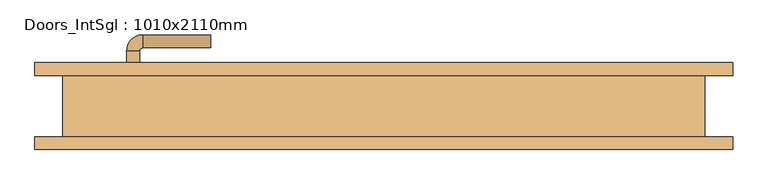
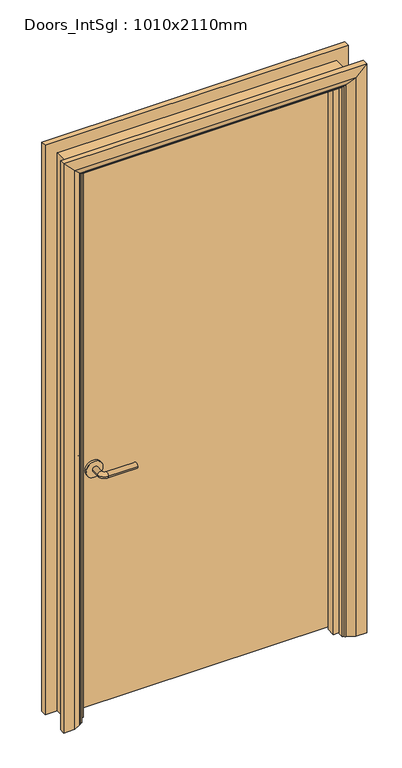
"""IFC4 building model written with IfcOpenShell, lengths in millimetres: door geometry, Doors_IntSgl : 1010x2110mm."""

from ifc_helpers import new_model, si_unit, point, frame, frame_2d, origin, place, context, project, spatial, polyline, circle_curve, ellipse_curve, trimmed, segment, composite_curve, outline, extrude, faceted_brep, source, transform, mapped, element, save
from ifc_brep_helpers import plane_surface, cylinder_surface, revolved_surface, advanced_brep


def doors_intsgl_1010x2110mm_9b3ab836(model_context):
    return source(origin(), model_context, "Body", "SolidModel", [
        advanced_brep(
        [(-398.0, 1.5, 900.0), (-378.0, 1.5, 900.0), (-378.0, -28.5, 900.0), (-398.0, -28.5, 900.0), (-373.0, -33.5, 900.0), (-373.0, -53.5, 900.0), (-268.0, -53.5, 900.0), (-268.0, -33.5, 900.0)],
        [
            (0, 1, circle_curve(frame((-388.0, 1.5, 900.0), z_axis=(0.0, 1.0, 0.0), x_axis=(1.0, 0.0, 0.0)), 10.0)),
            (1, 0, circle_curve(frame((-388.0, 1.5, 900.0), z_axis=(0.0, 1.0, 0.0), x_axis=(1.0, 0.0, 0.0)), 10.0)),
            (1, 2),
            (2, 3, circle_curve(frame((-388.0, -28.5, 900.0), z_axis=(0.0, 1.0, 0.0), x_axis=(1.0, 0.0, 0.0)), 10.0)),
            (3, 0),
            (3, 2, circle_curve(frame((-388.0, -28.5, 900.0), z_axis=(0.0, 1.0, 0.0), x_axis=(1.0, 0.0, 0.0)), 10.0)),
            (4, 5, circle_curve(frame((-373.0, -43.5, 900.0), z_axis=(-1.0, 0.0, 0.0), x_axis=(0.0, 1.0, 0.0)), 10.0)),
            (5, 3, circle_curve(frame((-373.0, -28.5, 900.0), z_axis=(0.0, 0.0, -1.0), x_axis=(-1.0, 0.0, 0.0)), 25.0)),
            (2, 4, circle_curve(frame((-373.0, -28.5, 900.0), z_axis=(0.0, 0.0, 1.0), x_axis=(-1.0, 0.0, 0.0)), 5.0)),
            (5, 4, circle_curve(frame((-373.0, -43.5, 900.0), z_axis=(-1.0, 0.0, 0.0), x_axis=(0.0, 1.0, 0.0)), 10.0)),
            (6, 7, circle_curve(frame((-268.0, -43.5, 900.0), z_axis=(1.0, 0.0, 0.0), x_axis=(0.0, 1.0, 0.0)), 10.0)),
            (7, 6, circle_curve(frame((-268.0, -43.5, 900.0), z_axis=(1.0, 0.0, 0.0), x_axis=(0.0, 1.0, 0.0)), 10.0)),
            (4, 7),
            (6, 5),
        ],
        [
            plane_surface(frame((-388.0, 1.5, 900.0), z_axis=(0.0, 1.0, 0.0), x_axis=(0.0, 0.0, 1.0))),
            cylinder_surface(frame((-388.0, 1.5, 900.0), z_axis=(0.0, 1.0, 0.0), x_axis=(1.0, 0.0, 0.0)), 10.0),
            revolved_surface(trimmed(ellipse_curve(frame((-388.0, -28.5, 900.0), z_axis=(0.0, -1.0, 0.0), x_axis=(1.0, 0.0, 0.0)), 10.0, 10.0), [point((-398.0, -28.5, 900.0))], [point((-378.0, -28.5, 900.0))], True, "CARTESIAN"), (-373.0, -28.5, 900.0), (0.0, 0.0, -1.0)),
            revolved_surface(trimmed(ellipse_curve(frame((-388.0, -28.5, 900.0), z_axis=(0.0, -1.0, 0.0), x_axis=(1.0, 0.0, 0.0)), 10.0, 10.0), [point((-378.0, -28.5, 900.0))], [point((-398.0, -28.5, 900.0))], True, "CARTESIAN"), (-373.0, -28.5, 900.0), (0.0, 0.0, -1.0)),
            plane_surface(frame((-268.0, -43.5, 900.0), z_axis=(1.0, 0.0, 0.0), x_axis=(0.0, 0.0, 1.0))),
            cylinder_surface(frame((-373.0, -43.5, 900.0), z_axis=(-1.0, 0.0, 0.0), x_axis=(0.0, 1.0, 0.0)), 10.0),
        ],
        [
            (0, [[1, 2]]),
            (1, [[3, 4, 5, -2]]),
            (1, [[-5, 6, -3, -1]]),
            (2, [[7, 8, -4, 9]]),
            (3, [[10, -9, -6, -8]]),
            (4, [[11, 12]]),
            (5, [[13, -11, 14, -7]]),
            (5, [[-14, -12, -13, -10]]),
        ],
    ),
        extrude(outline(composite_curve([segment(trimmed(circle_curve(frame_2d((900.0, -390.5)), 30.0), [point((900.0, -420.5))], [point((900.0, -360.5))], False, "CARTESIAN"), True, "CONTINUOUS"), segment(trimmed(circle_curve(frame_2d((900.0, -390.5)), 30.0), [point((900.0, -360.5))], [point((900.0, -420.5))], False, "CARTESIAN"), True, "CONTINUOUS")], self_intersect=False)), frame((0.0, 1.5, 0.0), z_axis=(0.0, 1.0, 0.0), x_axis=(0.0, 0.0, 1.0)), (0.0, 0.0, 1.0), 8.0),
        advanced_brep(
        [(-398.0, 55.5, 900.0), (-378.0, 55.5, 900.0), (-398.0, 85.5, 900.0), (-378.0, 85.5, 900.0), (-373.0, 90.5, 900.0), (-373.0, 110.5, 900.0), (-268.0, 110.5, 900.0), (-268.0, 90.5, 900.0)],
        [
            (0, 1, circle_curve(frame((-388.0, 55.5, 900.0), z_axis=(0.0, -1.0, 0.0), x_axis=(1.0, 0.0, 0.0)), 10.0)),
            (1, 0, circle_curve(frame((-388.0, 55.5, 900.0), z_axis=(0.0, -1.0, 0.0), x_axis=(1.0, 0.0, 0.0)), 10.0)),
            (0, 2),
            (2, 3, circle_curve(frame((-388.0, 85.5, 900.0), z_axis=(0.0, -1.0, 0.0), x_axis=(1.0, 0.0, 0.0)), 10.0)),
            (3, 1),
            (3, 2, circle_curve(frame((-388.0, 85.5, 900.0), z_axis=(0.0, -1.0, 0.0), x_axis=(1.0, 0.0, 0.0)), 10.0)),
            (4, 3, circle_curve(frame((-373.0, 85.5, 900.0), z_axis=(0.0, 0.0, 1.0), x_axis=(-1.0, 0.0, 0.0)), 5.0)),
            (2, 5, circle_curve(frame((-373.0, 85.5, 900.0), z_axis=(0.0, 0.0, -1.0), x_axis=(-1.0, 0.0, 0.0)), 25.0)),
            (5, 4, circle_curve(frame((-373.0, 100.5, 900.0), z_axis=(-1.0, 0.0, 0.0), x_axis=(0.0, -1.0, 0.0)), 10.0)),
            (4, 5, circle_curve(frame((-373.0, 100.5, 900.0), z_axis=(-1.0, 0.0, 0.0), x_axis=(0.0, -1.0, 0.0)), 10.0)),
            (6, 7, circle_curve(frame((-268.0, 100.5, 900.0), z_axis=(1.0, 0.0, 0.0), x_axis=(0.0, -1.0, 0.0)), 10.0)),
            (7, 6, circle_curve(frame((-268.0, 100.5, 900.0), z_axis=(1.0, 0.0, 0.0), x_axis=(0.0, -1.0, 0.0)), 10.0)),
            (5, 6),
            (7, 4),
        ],
        [
            plane_surface(frame((-388.0, 55.5, 900.0), z_axis=(0.0, -1.0, 0.0), x_axis=(0.0, 0.0, 1.0))),
            cylinder_surface(frame((-388.0, 55.5, 900.0), z_axis=(0.0, -1.0, 0.0), x_axis=(1.0, 0.0, 0.0)), 10.0),
            revolved_surface(trimmed(ellipse_curve(frame((-388.0, 85.5, 900.0), z_axis=(0.0, -1.0, 0.0), x_axis=(1.0, 0.0, 0.0)), 10.0, 10.0), [point((-398.0, 85.5, 900.0))], [point((-378.0, 85.5, 900.0))], True, "CARTESIAN"), (-373.0, 85.5, 900.0), (0.0, 0.0, -1.0)),
            revolved_surface(trimmed(ellipse_curve(frame((-388.0, 85.5, 900.0), z_axis=(0.0, -1.0, 0.0), x_axis=(1.0, 0.0, 0.0)), 10.0, 10.0), [point((-378.0, 85.5, 900.0))], [point((-398.0, 85.5, 900.0))], True, "CARTESIAN"), (-373.0, 85.5, 900.0), (0.0, 0.0, -1.0)),
            plane_surface(frame((-268.0, 100.5, 900.0), z_axis=(1.0, 0.0, 0.0), x_axis=(0.0, 0.0, 1.0))),
            cylinder_surface(frame((-373.0, 100.5, 900.0), z_axis=(-1.0, 0.0, 0.0), x_axis=(0.0, -1.0, 0.0)), 10.0),
        ],
        [
            (0, [[1, 2]]),
            (1, [[-1, 3, 4, 5]]),
            (1, [[-2, -5, 6, -3]]),
            (2, [[7, -4, 8, 9]]),
            (3, [[-8, -6, -7, 10]]),
            (4, [[11, 12]]),
            (5, [[-9, 13, -12, 14]]),
            (5, [[-10, -14, -11, -13]]),
        ],
    ),
        extrude(outline(composite_curve([segment(trimmed(circle_curve(frame_2d((900.0, -390.5)), 30.0), [point((900.0, -420.5))], [point((900.0, -360.5))], False, "CARTESIAN"), True, "CONTINUOUS"), segment(trimmed(circle_curve(frame_2d((900.0, -390.5)), 30.0), [point((900.0, -360.5))], [point((900.0, -420.5))], False, "CARTESIAN"), True, "CONTINUOUS")], self_intersect=False)), frame((0.0, 47.5, 0.0), z_axis=(0.0, 1.0, 0.0), x_axis=(0.0, 0.0, 1.0)), (0.0, 0.0, 1.0), 8.0),
        extrude(outline(polyline([(463.0, 9.5), (-463.0, 9.5), (-463.0, 47.5), (463.0, 47.5), (463.0, 9.5)])), frame((0.0, 0.0, 8.0), z_axis=(0.0, 0.0, 1.0), x_axis=(1.0, 0.0, 0.0)), (0.0, 0.0, 1.0), 2060.0),
        advanced_brep(
        [(540.0, 67.5, 0.0), (540.0, 47.5, 0.0), (470.0, 47.5, 0.0), (474.0, 53.5, 0.0), (500.0, 67.5, 0.0), (540.0, 67.5, 2145.0), (540.0, 47.5, 2145.0), (-540.0, 47.5, 2145.0), (-540.0, 47.5, 0.0), (-470.0, 47.5, 0.0), (-470.0, 47.5, 2075.0), (470.0, 47.5, 2075.0), (474.0, 53.5, 2079.0), (500.0, 67.5, 2105.0), (-500.0, 67.5, 2105.0), (-500.0, 67.5, 0.0), (-540.0, 67.5, 0.0), (-540.0, 67.5, 2145.0), (-474.0, 53.5, 2079.0), (-474.0, 53.5, 0.0)],
        [
            (0, 1),
            (1, 2),
            (2, 3, circle_curve(frame((478.0, 46.5, 0.0), z_axis=(0.0, 0.0, -1.0), x_axis=(1.0, 0.0, 0.0)), 8.0622577)),
            (3, 4),
            (4, 0),
            (0, 5),
            (5, 6),
            (6, 1),
            (6, 7),
            (7, 8),
            (8, 9),
            (9, 10),
            (10, 11),
            (11, 2),
            (11, 12, ellipse_curve(frame((478.0, 46.5, 2083.0), z_axis=(0.7071067811865475, 0.0, -0.7071067811865475), x_axis=(-0.7071067811865474, 0.0, -0.7071067811865476)), 11.4017543, 8.0622577)),
            (12, 3),
            (12, 13),
            (13, 4),
            (13, 14),
            (14, 15),
            (15, 16),
            (16, 17),
            (17, 5),
            (17, 7),
            (10, 18, ellipse_curve(frame((-478.0, 46.5, 2083.0), z_axis=(0.7071067811865475, 0.0, 0.7071067811865475), x_axis=(0.7071067811865476, 0.0, -0.7071067811865474)), 11.4017543, 8.0622577)),
            (18, 12),
            (18, 14),
            (15, 19),
            (19, 9, circle_curve(frame((-478.0, 46.5, 0.0), z_axis=(0.0, 0.0, -1.0), x_axis=(-1.0, 0.0, 0.0)), 8.0622577)),
            (8, 16),
            (19, 18),
        ],
        [
            plane_surface(frame((470.0, 47.5, 0.0), z_axis=(0.0, 0.0, -1.0), x_axis=(0.0, -1.0, 0.0))),
            plane_surface(frame((540.0, 67.5, 0.0), z_axis=(1.0, 0.0, 0.0), x_axis=(0.0, 0.0, 1.0))),
            plane_surface(frame((540.0, 47.5, 0.0), z_axis=(0.0, -1.0, 0.0), x_axis=(0.0, 0.0, 1.0))),
            cylinder_surface(frame((478.0, 46.5, 0.0), z_axis=(0.0, 0.0, -1.0), x_axis=(1.0, 0.0, 0.0)), 8.0622577),
            plane_surface(frame((474.0, 53.5, 0.0), z_axis=(-0.4740998230350126, 0.880471099922178, 0.0), x_axis=(0.0, 0.0, 1.0))),
            plane_surface(frame((500.0, 67.5, 0.0), z_axis=(0.0, 1.0, 0.0), x_axis=(0.0, 0.0, 1.0))),
            plane_surface(frame((540.0, 67.5, 2145.0), z_axis=(0.0, 0.0, 1.0), x_axis=(-1.0, 0.0, 0.0))),
            cylinder_surface(frame((470.0, 46.5, 2083.0), z_axis=(1.0, 0.0, 0.0), x_axis=(0.0, 0.0, 1.0)), 8.0622577),
            plane_surface(frame((474.0, 53.5, 2079.0), z_axis=(0.0, 0.8804710999221764, -0.4740998230350154), x_axis=(-1.0, 0.0, 0.0))),
            plane_surface(frame((-470.0, 47.5, 0.0), z_axis=(0.0, 0.0, -1.0), x_axis=(0.0, -1.0, 0.0))),
            plane_surface(frame((-540.0, 67.5, 2145.0), z_axis=(-1.0, 0.0, 0.0), x_axis=(0.0, 0.0, -1.0))),
            cylinder_surface(frame((-478.0, 46.5, 2075.0), z_axis=(0.0, 0.0, 1.0), x_axis=(-1.0, 0.0, 0.0)), 8.0622577),
            plane_surface(frame((-474.0, 53.5, 2079.0), z_axis=(0.47409982303501824, 0.8804710999221749, 0.0), x_axis=(0.0, 0.0, -1.0))),
        ],
        [
            (0, [[1, 2, 3, 4, 5]]),
            (1, [[-1, 6, 7, 8]]),
            (2, [[-2, -8, 9, 10, 11, 12, 13, 14]]),
            (3, [[-3, -14, 15, 16]]),
            (4, [[-4, -16, 17, 18]]),
            (5, [[-5, -18, 19, 20, 21, 22, 23, -6]]),
            (6, [[-7, -23, 24, -9]]),
            (7, [[-15, -13, 25, 26]]),
            (8, [[-17, -26, 27, -19]]),
            (9, [[-21, 28, 29, -11, 30]]),
            (10, [[-24, -22, -30, -10]]),
            (11, [[-25, -12, -29, 31]]),
            (12, [[-27, -31, -28, -20]]),
        ],
    ),
        extrude(outline(polyline([(0.0, -465.0), (0.0, -446.0), (2051.0, -446.0), (2051.0, 446.0), (0.0, 446.0), (0.0, 465.0), (2070.0, 465.0), (2070.0, -465.0), (0.0, -465.0)])), frame((0.0, -24.5, 0.0), z_axis=(0.0, 1.0, 0.0), x_axis=(0.0, 0.0, 1.0)), (0.0, 0.0, 1.0), 32.0),
        advanced_brep(
        [(-540.0, -67.5, 0.0), (-540.0, -47.5, 0.0), (-470.0, -47.5, 0.0), (-474.0, -53.5, 0.0), (-500.0, -67.5, 0.0), (-540.0, -67.5, 2145.0), (-540.0, -47.5, 2145.0), (-470.0, -47.5, 2075.0), (-474.0, -53.5, 2079.0), (-500.0, -67.5, 2105.0), (540.0, -67.5, 2145.0), (540.0, -47.5, 2145.0), (470.0, -47.5, 2075.0), (474.0, -53.5, 2079.0), (500.0, -67.5, 2105.0), (540.0, -67.5, 0.0), (500.0, -67.5, 0.0), (474.0, -53.5, 0.0), (470.0, -47.5, 0.0), (540.0, -47.5, 0.0)],
        [
            (0, 1),
            (1, 2),
            (2, 3, circle_curve(frame((-478.0, -46.5, 0.0), z_axis=(0.0, 0.0, -1.0), x_axis=(-1.0, 0.0, 0.0)), 8.0622577)),
            (3, 4),
            (4, 0),
            (0, 5),
            (5, 6),
            (6, 1),
            (6, 7),
            (7, 2),
            (7, 8, ellipse_curve(frame((-478.0, -46.5, 2083.0), z_axis=(-0.7071067811865475, 0.0, -0.7071067811865475), x_axis=(0.7071067811865474, 0.0, -0.7071067811865476)), 11.4017543, 8.0622577)),
            (8, 3),
            (8, 9),
            (9, 4),
            (9, 5),
            (5, 10),
            (10, 11),
            (11, 6),
            (11, 12),
            (12, 7),
            (12, 13, ellipse_curve(frame((478.0, -46.5, 2083.0), z_axis=(-0.7071067811865475, 0.0, 0.7071067811865475), x_axis=(-0.7071067811865476, 0.0, -0.7071067811865474)), 11.4017543, 8.0622577)),
            (13, 8),
            (13, 14),
            (14, 9),
            (14, 10),
            (15, 16),
            (16, 17),
            (17, 18, circle_curve(frame((478.0, -46.5, 0.0), z_axis=(0.0, 0.0, -1.0), x_axis=(1.0, 0.0, 0.0)), 8.0622577)),
            (18, 19),
            (19, 15),
            (10, 15),
            (19, 11),
            (18, 12),
            (17, 13),
            (16, 14),
        ],
        [
            plane_surface(frame((-470.0, -120.3010989, 0.0), z_axis=(0.0, 0.0, -1.0), x_axis=(1.0, 0.0, 0.0))),
            plane_surface(frame((-540.0, -67.5, 0.0), z_axis=(-1.0, 0.0, 0.0), x_axis=(0.0, 0.0, 1.0))),
            plane_surface(frame((-540.0, -47.5, 0.0), z_axis=(0.0, 1.0, 0.0), x_axis=(0.0, 0.0, 1.0))),
            cylinder_surface(frame((-478.0, -46.5, 0.0), z_axis=(0.0, 0.0, -1.0), x_axis=(-1.0, 0.0, 0.0)), 8.0622577),
            plane_surface(frame((-474.0, -53.5, 0.0), z_axis=(0.4740998230350183, -0.8804710999221749, 0.0), x_axis=(0.0, 0.0, 1.0))),
            plane_surface(frame((-500.0, -67.5, 0.0), z_axis=(0.0, -1.0, 0.0), x_axis=(0.0, 0.0, 1.0))),
            plane_surface(frame((-540.0, -67.5, 2145.0), z_axis=(0.0, 0.0, 1.0), x_axis=(1.0, 0.0, 0.0))),
            plane_surface(frame((-540.0, -47.5, 2145.0), z_axis=(0.0, 1.0, 0.0), x_axis=(1.0, 0.0, 0.0))),
            cylinder_surface(frame((-470.0, -46.5, 2083.0), z_axis=(-1.0, 0.0, 0.0), x_axis=(0.0, 0.0, 1.0)), 8.0622577),
            plane_surface(frame((-474.0, -53.5, 2079.0), z_axis=(0.0, -0.8804710999221749, -0.4740998230350183), x_axis=(1.0, 0.0, 0.0))),
            plane_surface(frame((-500.0, -67.5, 2105.0), z_axis=(0.0, -1.0, 0.0), x_axis=(1.0, 0.0, 0.0))),
            plane_surface(frame((470.0, -120.3010989, 0.0), z_axis=(0.0, 0.0, -1.0), x_axis=(-1.0, 0.0, 0.0))),
            plane_surface(frame((540.0, -67.5, 2145.0), z_axis=(1.0, 0.0, 0.0), x_axis=(0.0, 0.0, -1.0))),
            plane_surface(frame((540.0, -47.5, 2145.0), z_axis=(0.0, 1.0, 0.0), x_axis=(0.0, 0.0, -1.0))),
            cylinder_surface(frame((478.0, -46.5, 2075.0), z_axis=(0.0, 0.0, 1.0), x_axis=(1.0, 0.0, 0.0)), 8.0622577),
            plane_surface(frame((474.0, -53.5, 2079.0), z_axis=(-0.4740998230350183, -0.8804710999221749, 0.0), x_axis=(0.0, 0.0, -1.0))),
            plane_surface(frame((500.0, -67.5, 2105.0), z_axis=(0.0, -1.0, 0.0), x_axis=(0.0, 0.0, -1.0))),
        ],
        [
            (0, [[1, 2, 3, 4, 5]]),
            (1, [[-1, 6, 7, 8]]),
            (2, [[-2, -8, 9, 10]]),
            (3, [[-3, -10, 11, 12]]),
            (4, [[-4, -12, 13, 14]]),
            (5, [[-5, -14, 15, -6]]),
            (6, [[-7, 16, 17, 18]]),
            (7, [[-9, -18, 19, 20]]),
            (8, [[-11, -20, 21, 22]]),
            (9, [[-13, -22, 23, 24]]),
            (10, [[-15, -24, 25, -16]]),
            (11, [[26, 27, 28, 29, 30]]),
            (12, [[-17, 31, -30, 32]]),
            (13, [[-19, -32, -29, 33]]),
            (14, [[-21, -33, -28, 34]]),
            (15, [[-23, -34, -27, 35]]),
            (16, [[-25, -35, -26, -31]]),
        ],
    ),
        faceted_brep([(-465.0, 47.5, 0.0), (-465.0, -47.5, 0.0), (-497.0, -47.5, 0.0), (-497.0, 47.5, 0.0), (-465.0, 47.5, 2070.0), (-465.0, -47.5, 2070.0), (-497.0, -47.5, 2102.0), (-497.0, 47.5, 2102.0), (465.0, 47.5, 2070.0), (465.0, -47.5, 2070.0), (497.0, -47.5, 2102.0), (497.0, 47.5, 2102.0), (465.0, 47.5, 0.0), (497.0, 47.5, 0.0), (497.0, -47.5, 0.0), (465.0, -47.5, 0.0)], [[[0, 1, 2, 3]], [[1, 0, 4, 5]], [[2, 1, 5, 6]], [[3, 2, 6, 7]], [[0, 3, 7, 4]], [[5, 4, 8, 9]], [[6, 5, 9, 10]], [[7, 6, 10, 11]], [[4, 7, 11, 8]], [[12, 13, 14, 15]], [[9, 8, 12, 15]], [[10, 9, 15, 14]], [[11, 10, 14, 13]], [[8, 11, 13, 12]]]),
    ])


if __name__ == "__main__":
    model = new_model("IFC4")
    model_context = context("Model", 3, world=origin())
    ifc_project = project(units=[si_unit("LENGTHUNIT", "METRE", prefix="MILLI")], contexts=[model_context])
    site = spatial("IfcSite", under=ifc_project)
    building = spatial("IfcBuilding", under=site)
    placement = place(None, origin())
    doors_intsgl_1010x2110mm_shape = doors_intsgl_1010x2110mm_9b3ab836(model_context)
    element("IfcDoor", 1, ObjectType="Doors_IntSgl : 1010x2110mm", at=placement, inside=building, context=model_context, shape_type="MappedRepresentation", body=[
        mapped(doors_intsgl_1010x2110mm_shape, transform((0.0, 0.0, 0.0), x_axis=(1.0, 0.0, 0.0), y_axis=(0.0, 1.0, 0.0), z_axis=(0.0, 0.0, 1.0))),
    ])
    save(model, "model.ifc")

# Revit data of these elements
# Type "Doors_IntSgl : 1010x2110mm"
#   Construction Type Id = "MDOOR"
#   Type Mark = "43"
#   Type Comments = "Internal Single"
#   Operation = "SingleSwingRight"
#   Manufacturer = "Revit"
#   Keynote = "L20"
#   Description = "Internal Single Door"
#   Analytic Construction = "Metal"
#   UnderCut = 8 mm
#   Tolerance = 2 mm
#   Thickness = 38 mm
#   Thermal Resistance (R) = 0.270117 (m²·K)/W
#   Structural Tolerance = 8 mm
#   StopDepth = 32 mm
#   Stop Thickness = 19 mm
#   Rough Width = 1010 mm
#   Rough Height = 2110 mm
#   Height to Top Lock Rail = 1000 mm
#   Heat Transfer Coefficient (U) = 3.7021 W/(m²·K)
#   Handle Z Distance = 900 mm
#   Handle X Distance = 75 mm
#   Frame Thickness = 32 mm
#   Door Panel Width = 926 mm
#   Door Panel Thickness = 38 mm
#   Door Panel Offset = 0 mm
#   Height = 2110 mm
#   Width = 1010 mm
#   Door Panel Height = 2060 mm
#   Architrave Setback = 5 mm
#   Vis - Ironmongery = yes
#   Material Ironmongery = Door - Handle
#   Material Frame = Door - Frame/Mullion (1)
#   Material Door = Door - Panel
#   Material Architrave = Door - Architrave
#   Visual Light Transmittance = 0
#   Solar Heat Gain Coefficient = 0
#   Function = (empty or 0)
#   Wall Closure = (empty or 0)
# Element 1 (IfcDoor, "Doors_IntSgl : 1010x2110mm")
#   Materials on its faces: "Door - Architrave", "Door - Handle", "Door - Frame/Mullion (1)", "Door - Panel"
# Materials
#   "Door - Handle": class "Miscellaneous", colour RGB 0 0 0, transparency 0, Keynote = "P21", Cost = 0
#   "Door - Frame/Mullion (1)": class "Wood", colour RGB 212 179 113, transparency 0, Keynote = "L20", Cost = 0
#   "Door - Panel": class "Wood", colour RGB 210 159 95, transparency 0, Keynote = "L20", Cost = 0
#   "Door - Architrave": class "Wood", colour RGB 154 90 5, transparency 0, Keynote = "P20", Cost = 0
